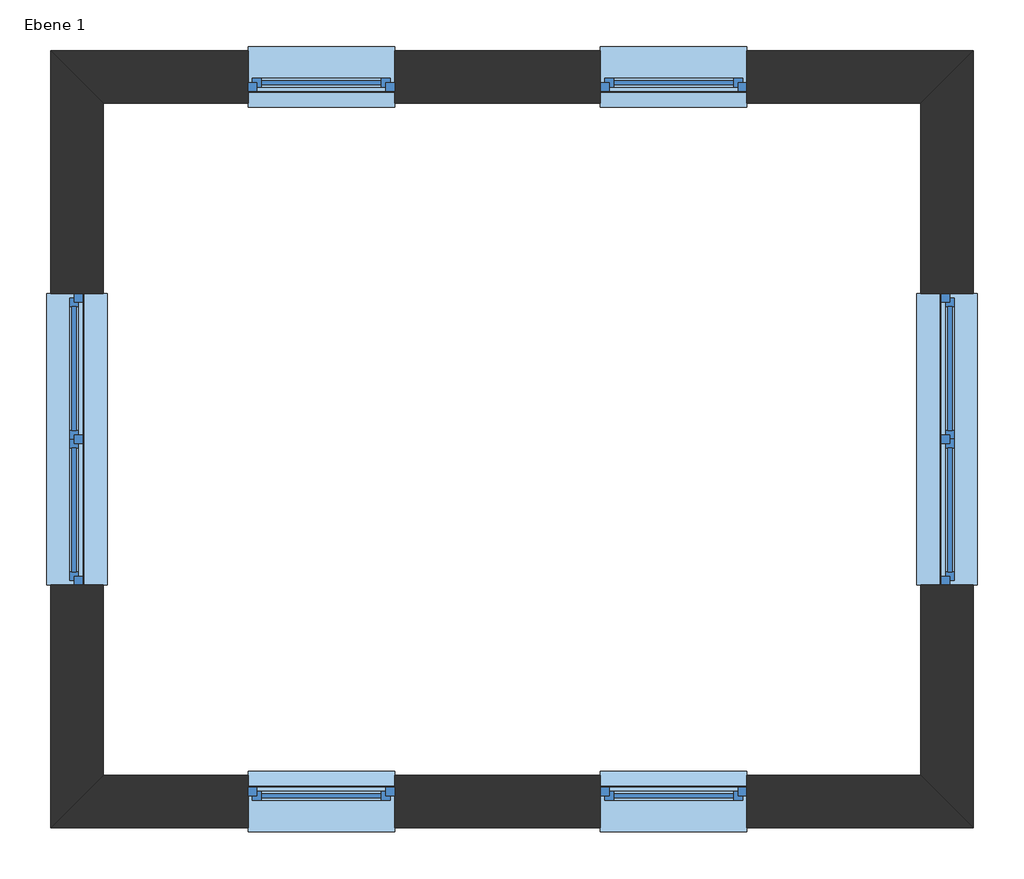
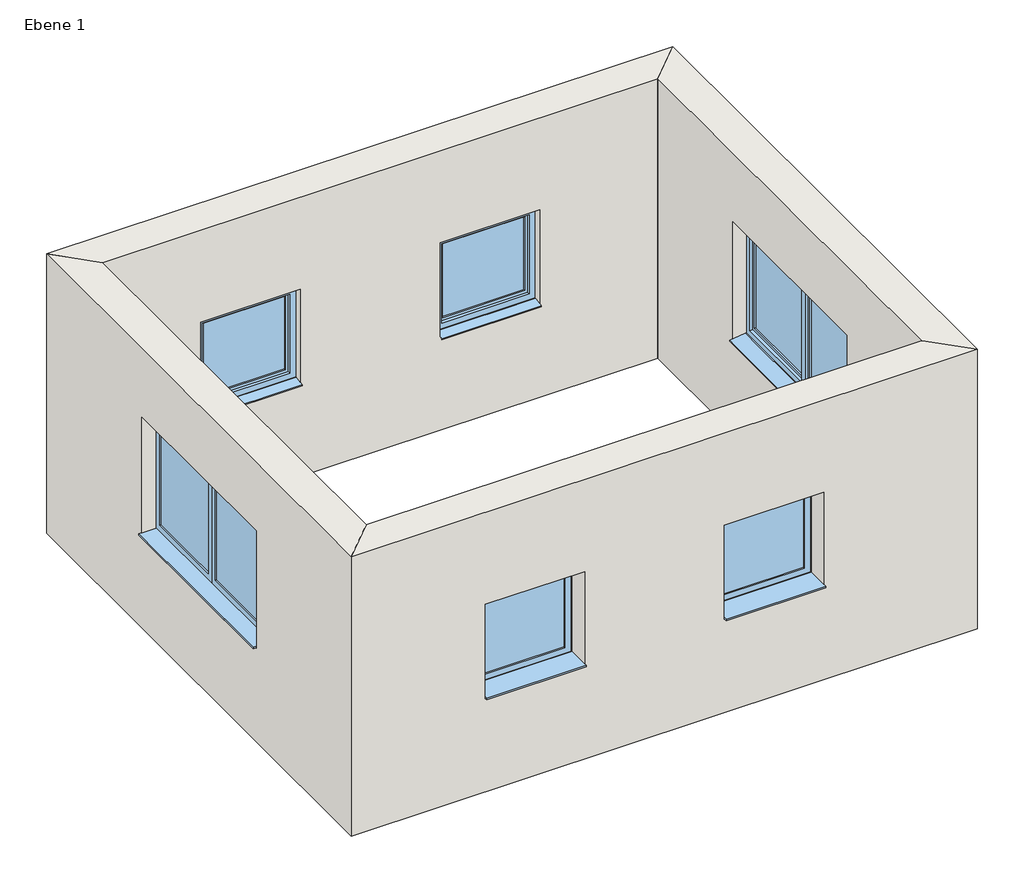
# One storey: 6 windows, 4 walls.
"""IFC4 building model written with IfcOpenShell, lengths in millimetres."""

import ifcopenshell
import ifcopenshell.guid

model = None  # the IFC model being written
_history = None  # IfcOwnerHistory: only IFC2X3 demands one
_inside = {}  # id of a spatial element -> (the spatial element, [elements in it])
_under = {}  # id of a project, library or spatial element -> (it, [spatial elements below it])
_declared = {}  # id of a project -> (the project, [libraries it declares])
_typed = {}  # id of a type object -> (the type object, [elements of that type])
_made_of = {}  # id of a material, layer set ... -> (it, [elements and type objects made of it])


def new_model(schema):
    """Start an empty IFC model of exactly this schema.

    Asked for "IFC4X3", IfcOpenShell would pick the latest addendum, in which some entities
    have other attributes; the version numbers below select the first issue.
    IFC2X3 requires an IfcOwnerHistory on every rooted entity: one is made here for all.
    """
    global model, _history
    if schema == "IFC4X3":
        model = ifcopenshell.file(schema_version=(4, 3, 0, 0))
    else:
        model = ifcopenshell.file(schema=schema)
    _inside.clear()
    _under.clear()
    _declared.clear()
    _typed.clear()
    _made_of.clear()
    _history = None
    if model.schema == "IFC2X3":
        org = make("IfcOrganization", Name="unknown")
        user = make(
            "IfcPersonAndOrganization",
            ThePerson=make("IfcPerson", FamilyName="unknown"),
            TheOrganization=org,
        )
        app = make(
            "IfcApplication",
            ApplicationDeveloper=org,
            Version="unknown",
            ApplicationFullName="unknown",
            ApplicationIdentifier="unknown",
        )
        _history = make(
            "IfcOwnerHistory",
            OwningUser=user,
            OwningApplication=app,
            ChangeAction="ADDED",
            CreationDate=0,
        )
    return model


def make(cls, **values):
    """One entity of the class cls with the attributes given. An attribute that is None is left unset."""
    return model.create_entity(
        cls, **{name: value for name, value in values.items() if value is not None}
    )


def rooted(cls, **values):
    """An entity with a GlobalId (a new one), such as an element, a storey or a relation."""
    return make(cls, GlobalId=ifcopenshell.guid.new(), OwnerHistory=_history, **values)


def si_unit(unit_type, name, prefix=None):
    """IfcSIUnit, for example si_unit("LENGTHUNIT", "METRE", prefix="MILLI")."""
    return make("IfcSIUnit", UnitType=unit_type, Prefix=prefix, Name=name)


def assignment(units):
    """IfcUnitAssignment: the units of a project."""
    return None if units is None else make("IfcUnitAssignment", Units=units)


def point(xyz):
    """IfcCartesianPoint."""
    return None if xyz is None else make("IfcCartesianPoint", Coordinates=xyz)


def direction(xyz):
    """IfcDirection."""
    return None if xyz is None else make("IfcDirection", DirectionRatios=xyz)


def frame(location, z_axis=None, x_axis=None):
    """IfcAxis2Placement3D, a coordinate frame: its origin and axes. An axis left out is left unset."""
    return make(
        "IfcAxis2Placement3D",
        Location=point(location),
        Axis=direction(z_axis),
        RefDirection=direction(x_axis),
    )


def origin():
    """The frame at (0, 0, 0) with its axes left unset."""
    return frame((0.0, 0.0, 0.0))


def place(relative_to, where):
    """IfcLocalPlacement: puts the frame where relative to a parent placement (None: the world)."""
    return make(
        "IfcLocalPlacement", PlacementRelTo=relative_to, RelativePlacement=where
    )


def context(
    kind, dimensions, precision=None, world=None, true_north=None, identifier=None
):
    """IfcGeometricRepresentationContext, for example the 3D "Model" context."""
    return make(
        "IfcGeometricRepresentationContext",
        ContextIdentifier=identifier,
        ContextType=kind,
        CoordinateSpaceDimension=dimensions,
        Precision=precision,
        WorldCoordinateSystem=world,
        TrueNorth=true_north,
    )


def project(units=None, contexts=None):
    """IfcProject with its units and contexts."""
    return rooted(
        "IfcProject",
        Name="project",
        RepresentationContexts=contexts,
        UnitsInContext=assignment(units),
    )


def spatial(cls, under=None, at=None, **own):
    """A site, building, storey or space (cls), placed at a placement, below another one or the project."""
    s = rooted(cls, ObjectPlacement=at, **own)
    if under is not None:
        _under.setdefault(under.id(), (under, []))[1].append(s)
    return s


def polyline(points):
    """IfcPolyline through the points."""
    return make("IfcPolyline", Points=[point(p) for p in points])


def outline(outer, holes=None, kind="AREA"):
    """IfcArbitraryClosedProfileDef: a profile drawn as a closed curve; with holes, ...WithVoids."""
    if holes is None:
        return make("IfcArbitraryClosedProfileDef", ProfileType=kind, OuterCurve=outer)
    return make(
        "IfcArbitraryProfileDefWithVoids",
        ProfileType=kind,
        OuterCurve=outer,
        InnerCurves=holes,
    )


def extrude(swept, where, along, depth):
    """IfcExtrudedAreaSolid: the profile swept, set in the frame where, extruded along a direction by depth."""
    return make(
        "IfcExtrudedAreaSolid",
        SweptArea=swept,
        Position=where,
        ExtrudedDirection=direction(along),
        Depth=depth,
    )


def faces_of(points, faces, orient=None, outer=None):
    """IfcFace entities. A face is a list of loops; a loop is a list of indices into points, from 0.

    orient and outer hold one flag for each loop. By default every Orientation is true, the
    first loop of a face is its IfcFaceOuterBound and the others are IfcFaceBound.
    """
    made = []
    for i, loops in enumerate(faces):
        bounds = []
        for j, loop in enumerate(loops):
            is_outer = j == 0 if outer is None else outer[i][j]
            bounds.append(
                make(
                    "IfcFaceOuterBound" if is_outer else "IfcFaceBound",
                    Bound=make("IfcPolyLoop", Polygon=[points[k] for k in loop]),
                    Orientation=True if orient is None else orient[i][j],
                )
            )
        made.append(make("IfcFace", Bounds=bounds))
    return made


def faceted_brep(points, faces, orient=None, outer=None, voids=None):
    """IfcFacetedBrep: a solid bounded by flat faces; with voids (closed shells), ...WithVoids."""
    shared = [point(p) for p in points]
    hull = make("IfcClosedShell", CfsFaces=faces_of(shared, faces, orient, outer))
    if voids is None:
        return make("IfcFacetedBrep", Outer=hull)
    return make(
        "IfcFacetedBrepWithVoids",
        Outer=hull,
        Voids=[
            make(cls, CfsFaces=faces_of(shared, fs, o, b)) for cls, fs, o, b in voids
        ],
    )


def shape(context_of_items, identifier, shape_type, items):
    """IfcShapeRepresentation: the items that make up one representation, for example the "Body"."""
    return make(
        "IfcShapeRepresentation",
        ContextOfItems=context_of_items,
        RepresentationIdentifier=identifier,
        RepresentationType=shape_type,
        Items=items,
    )


def source(mapping_origin, context_of_items, identifier, shape_type, items):
    """IfcRepresentationMap: a shape defined once, which mapped items show again and again."""
    return make(
        "IfcRepresentationMap",
        MappingOrigin=mapping_origin,
        MappedRepresentation=shape(context_of_items, identifier, shape_type, items),
    )


def transform(
    local_origin,
    x_axis=None,
    y_axis=None,
    z_axis=None,
    scale=None,
    scale2=None,
    scale3=None,
    uniform=True,
):
    """IfcCartesianTransformationOperator3D, or its non-uniform kind. x_axis, y_axis, z_axis: its Axis1, 2, 3."""
    if uniform:
        return make(
            "IfcCartesianTransformationOperator3D",
            Axis1=direction(x_axis),
            Axis2=direction(y_axis),
            LocalOrigin=point(local_origin),
            Scale=scale,
            Axis3=direction(z_axis),
        )
    return make(
        "IfcCartesianTransformationOperator3DnonUniform",
        Axis1=direction(x_axis),
        Axis2=direction(y_axis),
        LocalOrigin=point(local_origin),
        Scale=scale,
        Axis3=direction(z_axis),
        Scale2=scale2,
        Scale3=scale3,
    )


def mapped(mapping_source, mapping_target):
    """IfcMappedItem: shows the shape of a source again, moved by a transform."""
    return make(
        "IfcMappedItem", MappingSource=mapping_source, MappingTarget=mapping_target
    )


def made_of(thing, what):
    """Note that an element or type object is made of a material, layer set ...; save() writes the relation."""
    if what is not None:
        _made_of.setdefault(what.id(), (what, []))[1].append(thing)
    return thing


def element(
    cls,
    number,
    at=None,
    inside=None,
    cuts=None,
    type_object=None,
    material=None,
    context=None,
    identifier="Body",
    shape_type=None,
    held_by="IfcProductDefinitionShape",
    body=None,
    shapes=None,
    **own,
):
    """One element of the class cls, such as IfcWall. Its Tag is "e" and its number.

    at: its placement. inside: the storey or other place that contains it. cuts: it is an
    opening in that element (IfcRelVoidsElement). A single representation is given by context,
    identifier, shape_type and body (its items); several are given by shapes. held_by: the class
    of the entity that holds the representations. save() writes the other relations.
    """
    e = rooted(cls, Tag="e%d" % number, ObjectPlacement=at, **own)
    if body is not None:
        shapes = [shape(context, identifier, shape_type, body)]
    if shapes is not None:
        e.Representation = make(held_by, Representations=shapes)
    if inside is not None:
        _inside.setdefault(inside.id(), (inside, []))[1].append(e)
    if cuts is not None:
        rooted(
            "IfcRelVoidsElement", RelatingBuildingElement=cuts, RelatedOpeningElement=e
        )
    if type_object is not None:
        _typed.setdefault(type_object.id(), (type_object, []))[1].append(e)
    return made_of(e, material)


def aggregate(whole, parts):
    """IfcRelAggregates: a whole, such as a stair, and the parts it consists of."""
    return rooted("IfcRelAggregates", RelatingObject=whole, RelatedObjects=parts)


def save(model, path):
    """Write the relations noted so far, then the file.

    IfcRelAggregates (storeys below a building ...), IfcRelContainedInSpatialStructure (elements
    in a storey), IfcRelDefinesByType, IfcRelAssociatesMaterial and IfcRelDeclares: one each for
    every whole, place, type object, material and project.
    """
    for whole, parts in _under.values():
        aggregate(whole, parts)
    for where, things in _inside.values():
        rooted(
            "IfcRelContainedInSpatialStructure",
            RelatedElements=things,
            RelatingStructure=where,
        )
    for kind, things in _typed.values():
        rooted("IfcRelDefinesByType", RelatedObjects=things, RelatingType=kind)
    for what, things in _made_of.values():
        rooted("IfcRelAssociatesMaterial", RelatedObjects=things, RelatingMaterial=what)
    for by, libraries in _declared.values():
        rooted("IfcRelDeclares", RelatingContext=by, RelatedDefinitions=libraries)
    model.write(path)


def fenster_1_flg_variabel_fenster_1_flg_variabel_3_8a378bad(model_context):
    return source(origin(), model_context, "Body", "SolidModel", [
        extrude(outline(polyline([(2010.0, 505.0), (2010.0, -505.0), (1000.0, -505.0), (1000.0, 505.0), (2010.0, 505.0)]), holes=[polyline([(1930.0, 445.0), (1080.0, 445.0), (1080.0, -445.0), (1930.0, -445.0), (1930.0, 445.0)])]), frame((0.0, 40.0, 0.0), z_axis=(0.0, 1.0, 0.0), x_axis=(0.0, 0.0, 1.0)), (0.0, 0.0, 1.0), 60.0),
        faceted_brep([(475.0, 40.0, 1960.0), (475.0, 10.0, 1960.0), (475.0, 10.0, 1050.0), (475.0, 40.0, 1050.0), (-475.0, 10.0, 1960.0), (-475.0, 10.0, 1050.0), (415.0, 10.0, 1110.0), (-415.0, 10.0, 1110.0), (-415.0, 10.0, 1900.0), (415.0, 10.0, 1900.0), (-475.0, 40.0, 1050.0), (-475.0, 40.0, 1960.0), (445.0, 40.0, 1930.0), (-445.0, 40.0, 1930.0), (-445.0, 40.0, 1080.0), (445.0, 40.0, 1080.0), (445.0, 70.0, 1930.0), (445.0, 70.0, 1080.0), (-445.0, 70.0, 1080.0), (-445.0, 70.0, 1930.0), (415.0, 70.0, 1900.0), (-415.0, 70.0, 1900.0), (-415.0, 70.0, 1110.0), (415.0, 70.0, 1110.0)], [[[0, 1, 2, 3]], [[1, 4, 5, 2], [6, 7, 8, 9]], [[3, 2, 5, 10]], [[3, 10, 11, 0], [12, 13, 14, 15]], [[16, 12, 15, 17]], [[17, 15, 14, 18]], [[17, 18, 19, 16], [20, 21, 22, 23]], [[9, 20, 23, 6]], [[6, 23, 22, 7]], [[10, 5, 4, 11]], [[18, 14, 13, 19]], [[7, 22, 21, 8]], [[11, 4, 1, 0]], [[19, 13, 12, 16]], [[8, 21, 20, 9]]]),
        extrude(outline(polyline([(-505.0, -210.0), (-505.0, 40.0), (505.0, 40.0), (505.0, -210.0), (-505.0, -210.0)])), frame((0.0, 0.0, 1005.0), z_axis=(0.0, 0.0, 1.0), x_axis=(1.0, 0.0, 0.0)), (0.0, 0.0, 1.0), 15.0),
        extrude(outline(polyline([(110.0221543, 1020.0), (210.0, 1000.0), (210.0, 990.0), (208.0, 990.0), (208.0, 998.3604634), (109.8240723, 1018.0), (100.0, 1018.0), (100.0, 1020.0), (110.0221543, 1020.0)])), frame((-505.0, 0.0, 0.0), z_axis=(1.0, 0.0, 0.0), x_axis=(0.0, 1.0, 0.0)), (0.0, 0.0, 1.0), 1010.0),
        extrude(outline(polyline([(415.0, 25.0), (-415.0, 25.0), (-415.0, 55.0), (415.0, 55.0), (415.0, 25.0)])), frame((0.0, 0.0, 1110.0), z_axis=(0.0, 0.0, 1.0), x_axis=(1.0, 0.0, 0.0)), (0.0, 0.0, 1.0), 790.0),
    ])


def fenster_2_flg_variabel_fenster_2_flg_variabel_3_03287464(model_context):
    return source(origin(), model_context, "Body", "SolidModel", [
        extrude(outline(polyline([(60.0, -5.0), (915.0, -5.0), (915.0, -35.0), (60.0, -35.0), (60.0, -5.0)])), frame((0.0, 0.0, 1110.0), z_axis=(0.0, 0.0, 1.0), x_axis=(1.0, 0.0, 0.0)), (0.0, 0.0, 1.0), 1040.0),
        extrude(outline(polyline([(-915.0, -5.0), (-60.0, -5.0), (-60.0, -35.0), (-915.0, -35.0), (-915.0, -5.0)])), frame((0.0, 0.0, 1110.0), z_axis=(0.0, 0.0, 1.0), x_axis=(1.0, 0.0, 0.0)), (0.0, 0.0, 1.0), 1040.0),
        extrude(outline(polyline([(-1005.0, -210.0), (-1005.0, -20.0), (1005.0, -20.0), (1005.0, -210.0), (-1005.0, -210.0)])), frame((0.0, 0.0, 1005.0), z_axis=(0.0, 0.0, 1.0), x_axis=(1.0, 0.0, 0.0)), (0.0, 0.0, 1.0), 15.0),
        extrude(outline(polyline([(50.0221543, 1020.0), (210.0, 1000.0), (210.0, 990.0), (208.0, 990.0), (208.0, 998.3604634), (49.8240723, 1018.0), (40.0, 1018.0), (40.0, 1020.0), (50.0221543, 1020.0)])), frame((-1005.0, 0.0, 0.0), z_axis=(1.0, 0.0, 0.0), x_axis=(0.0, 1.0, 0.0)), (0.0, 0.0, 1.0), 2010.0),
        extrude(outline(polyline([(30.0, -20.0), (-30.0, -20.0), (-30.0, 40.0), (30.0, 40.0), (30.0, -20.0)])), frame((0.0, 0.0, 1080.0), z_axis=(0.0, 0.0, 1.0), x_axis=(1.0, 0.0, 0.0)), (0.0, 0.0, 1.0), 1100.0),
        extrude(outline(polyline([(2260.0, -1005.0), (1000.0, -1005.0), (1000.0, 1005.0), (2260.0, 1005.0), (2260.0, -1005.0)]), holes=[polyline([(2180.0, -945.0), (2180.0, 945.0), (1080.0, 945.0), (1080.0, -945.0), (2180.0, -945.0)])]), frame((0.0, -20.0, 0.0), z_axis=(0.0, 1.0, 0.0), x_axis=(0.0, 0.0, 1.0)), (0.0, 0.0, 1.0), 60.0),
        faceted_brep([(-945.0, -20.0, 1080.0), (-945.0, 10.0, 1080.0), (-30.0, 10.0, 1080.0), (-30.0, -20.0, 1080.0), (-30.0, 10.0, 2180.0), (-30.0, -20.0, 2180.0), (-945.0, 10.0, 2180.0), (-60.0, 10.0, 2150.0), (-915.0, 10.0, 2150.0), (-915.0, 10.0, 1110.0), (-60.0, 10.0, 1110.0), (0.0, -20.0, 1050.0), (-975.0, -20.0, 1050.0), (-975.0, -20.0, 2210.0), (0.0, -20.0, 2210.0), (-945.0, -20.0, 2180.0), (-975.0, -50.0, 1050.0), (0.0, -50.0, 1050.0), (0.0, -50.0, 2210.0), (-975.0, -50.0, 2210.0), (-60.0, -50.0, 1110.0), (-915.0, -50.0, 1110.0), (-915.0, -50.0, 2150.0), (-60.0, -50.0, 2150.0)], [[[0, 1, 2, 3]], [[3, 2, 4, 5]], [[2, 1, 6, 4], [7, 8, 9, 10]], [[11, 12, 13, 14], [5, 15, 0, 3]], [[16, 12, 11, 17]], [[17, 11, 14, 18]], [[18, 19, 16, 17], [20, 21, 22, 23]], [[9, 21, 20, 10]], [[10, 20, 23, 7]], [[15, 6, 1, 0]], [[19, 13, 12, 16]], [[8, 22, 21, 9]], [[5, 4, 6, 15]], [[18, 14, 13, 19]], [[7, 23, 22, 8]]]),
        faceted_brep([(30.0, -20.0, 1080.0), (30.0, 10.0, 1080.0), (945.0, 10.0, 1080.0), (945.0, -20.0, 1080.0), (945.0, 10.0, 2180.0), (945.0, -20.0, 2180.0), (30.0, 10.0, 2180.0), (915.0, 10.0, 2150.0), (60.0, 10.0, 2150.0), (60.0, 10.0, 1110.0), (915.0, 10.0, 1110.0), (975.0, -20.0, 1050.0), (0.0, -20.0, 1050.0), (0.0, -20.0, 2210.0), (975.0, -20.0, 2210.0), (30.0, -20.0, 2180.0), (0.0, -50.0, 1050.0), (975.0, -50.0, 1050.0), (975.0, -50.0, 2210.0), (0.0, -50.0, 2210.0), (915.0, -50.0, 1110.0), (60.0, -50.0, 1110.0), (60.0, -50.0, 2150.0), (915.0, -50.0, 2150.0)], [[[0, 1, 2, 3]], [[3, 2, 4, 5]], [[2, 1, 6, 4], [7, 8, 9, 10]], [[11, 12, 13, 14], [5, 15, 0, 3]], [[16, 12, 11, 17]], [[17, 11, 14, 18]], [[18, 19, 16, 17], [20, 21, 22, 23]], [[9, 21, 20, 10]], [[10, 20, 23, 7]], [[15, 6, 1, 0]], [[19, 13, 12, 16]], [[8, 22, 21, 9]], [[5, 4, 6, 15]], [[18, 14, 13, 19]], [[7, 23, 22, 8]]]),
    ])


model = new_model("IFC4")

# Units and contexts
model_context = context("Model", 3, world=origin())
ifc_project = project(units=[si_unit("LENGTHUNIT", "METRE", prefix="MILLI")], contexts=[model_context])

# Site, building, storey
site = spatial("IfcSite", under=ifc_project)
building = spatial("IfcBuilding", under=site)
storey = spatial("IfcBuildingStorey", under=building, Name="Ebene 1", Elevation=3000.0)

# Walls
placement = place(None, origin())
element("IfcWall", 1, ObjectType="MW 24.0 WD 12.0", at=placement, inside=storey, context=model_context, shape_type="Brep", body=[
    faceted_brep([(-6003.5987005, 5004.2257101, 3000.0), (-363.5987005, 5004.2257101, 3000.0), (-363.5987005, 5004.2257101, 6000.0), (-6003.5987005, 5004.2257101, 6000.0), (-1563.5987005, 5004.2257101, 4000.0), (-2573.5987005, 5004.2257101, 4000.0), (-2573.5987005, 5004.2257101, 5010.0), (-1563.5987005, 5004.2257101, 5010.0), (-3993.5987005, 5004.2257101, 4000.0), (-5003.5987005, 5004.2257101, 4000.0), (-5003.5987005, 5004.2257101, 5010.0), (-3993.5987005, 5004.2257101, 5010.0), (-6363.5987005, 5364.2257101, 3000.0), (-6363.5987005, 5364.2257101, 6000.0), (-3.5987005, 5364.2257101, 6000.0), (-3.5987005, 5364.2257101, 3000.0), (-1563.5987005, 5364.2257101, 4000.0), (-1563.5987005, 5364.2257101, 5010.0), (-2573.5987005, 5364.2257101, 5010.0), (-2573.5987005, 5364.2257101, 4000.0), (-3993.5987005, 5364.2257101, 4000.0), (-3993.5987005, 5364.2257101, 5010.0), (-5003.5987005, 5364.2257101, 5010.0), (-5003.5987005, 5364.2257101, 4000.0)], [[[0, 1, 2, 3], [4, 5, 6, 7], [8, 9, 10, 11]], [[12, 13, 14, 15], [16, 17, 18, 19], [20, 21, 22, 23]], [[1, 0, 12, 15]], [[3, 2, 14, 13]], [[2, 1, 15, 14]], [[0, 3, 13, 12]], [[17, 16, 4, 7]], [[18, 17, 7, 6]], [[19, 18, 6, 5]], [[16, 19, 5, 4]], [[21, 20, 8, 11]], [[22, 21, 11, 10]], [[23, 22, 10, 9]], [[20, 23, 9, 8]]]),
])
element("IfcWall", 2, ObjectType="MW 24.0 WD 12.0", at=placement, inside=storey, context=model_context, shape_type="Brep", body=[
    faceted_brep([(-363.5987005, 5004.2257101, 3000.0), (-363.5987005, 364.2257101, 3000.0), (-363.5987005, 364.2257101, 6000.0), (-363.5987005, 5004.2257101, 6000.0), (-363.5987005, 1679.2257101, 4000.0), (-363.5987005, 3689.2257101, 4000.0), (-363.5987005, 3689.2257101, 5260.0), (-363.5987005, 1679.2257101, 5260.0), (-3.5987005, 5364.2257101, 3000.0), (-3.5987005, 5364.2257101, 6000.0), (-3.5987005, 4.2257101, 6000.0), (-3.5987005, 4.2257101, 3000.0), (-3.5987005, 1679.2257101, 4000.0), (-3.5987005, 1679.2257101, 5260.0), (-3.5987005, 3689.2257101, 5260.0), (-3.5987005, 3689.2257101, 4000.0)], [[[0, 1, 2, 3], [4, 5, 6, 7]], [[8, 9, 10, 11], [12, 13, 14, 15]], [[1, 0, 8, 11]], [[3, 2, 10, 9]], [[0, 3, 9, 8]], [[2, 1, 11, 10]], [[13, 12, 4, 7]], [[14, 13, 7, 6]], [[15, 14, 6, 5]], [[12, 15, 5, 4]]]),
])
element("IfcWall", 3, ObjectType="MW 24.0 WD 12.0", at=placement, inside=storey, context=model_context, shape_type="Brep", body=[
    faceted_brep([(-363.5987005, 364.2257101, 3000.0), (-6003.5987005, 364.2257101, 3000.0), (-6003.5987005, 364.2257101, 6000.0), (-363.5987005, 364.2257101, 6000.0), (-2573.5987005, 364.2257101, 4000.0), (-1563.5987005, 364.2257101, 4000.0), (-1563.5987005, 364.2257101, 5010.0), (-2573.5987005, 364.2257101, 5010.0), (-5003.5987005, 364.2257101, 4000.0), (-3993.5987005, 364.2257101, 4000.0), (-3993.5987005, 364.2257101, 5010.0), (-5003.5987005, 364.2257101, 5010.0), (-3.5987005, 4.2257101, 3000.0), (-3.5987005, 4.2257101, 6000.0), (-6363.5987005, 4.2257101, 6000.0), (-6363.5987005, 4.2257101, 3000.0), (-2573.5987005, 4.2257101, 4000.0), (-2573.5987005, 4.2257101, 5010.0), (-1563.5987005, 4.2257101, 5010.0), (-1563.5987005, 4.2257101, 4000.0), (-5003.5987005, 4.2257101, 4000.0), (-5003.5987005, 4.2257101, 5010.0), (-3993.5987005, 4.2257101, 5010.0), (-3993.5987005, 4.2257101, 4000.0)], [[[0, 1, 2, 3], [4, 5, 6, 7], [8, 9, 10, 11]], [[12, 13, 14, 15], [16, 17, 18, 19], [20, 21, 22, 23]], [[1, 0, 12, 15]], [[3, 2, 14, 13]], [[0, 3, 13, 12]], [[2, 1, 15, 14]], [[17, 16, 4, 7]], [[18, 17, 7, 6]], [[19, 18, 6, 5]], [[16, 19, 5, 4]], [[21, 20, 8, 11]], [[22, 21, 11, 10]], [[23, 22, 10, 9]], [[20, 23, 9, 8]]]),
])
element("IfcWall", 4, ObjectType="MW 24.0 WD 12.0", at=placement, inside=storey, context=model_context, shape_type="Brep", body=[
    faceted_brep([(-6003.5987005, 364.2257101, 3000.0), (-6003.5987005, 5004.2257101, 3000.0), (-6003.5987005, 5004.2257101, 6000.0), (-6003.5987005, 364.2257101, 6000.0), (-6003.5987005, 3689.2257101, 4000.0), (-6003.5987005, 1679.2257101, 4000.0), (-6003.5987005, 1679.2257101, 5260.0), (-6003.5987005, 3689.2257101, 5260.0), (-6363.5987005, 4.2257101, 3000.0), (-6363.5987005, 4.2257101, 6000.0), (-6363.5987005, 5364.2257101, 6000.0), (-6363.5987005, 5364.2257101, 3000.0), (-6363.5987005, 3689.2257101, 4000.0), (-6363.5987005, 3689.2257101, 5260.0), (-6363.5987005, 1679.2257101, 5260.0), (-6363.5987005, 1679.2257101, 4000.0)], [[[0, 1, 2, 3], [4, 5, 6, 7]], [[8, 9, 10, 11], [12, 13, 14, 15]], [[1, 0, 8, 11]], [[3, 2, 10, 9]], [[2, 1, 11, 10]], [[0, 3, 9, 8]], [[13, 12, 4, 7]], [[14, 13, 7, 6]], [[15, 14, 6, 5]], [[12, 15, 5, 4]]]),
])

# Windows
fenster_1_flg_variabel_fenster_1_flg_variabel_3_shape = fenster_1_flg_variabel_fenster_1_flg_variabel_3_8a378bad(model_context)
element("IfcWindow", 5, ObjectType="Fenster 1-flg - Variabel : Fenster 1-flg - Variabel 3", at=placement, inside=storey, context=model_context, shape_type="MappedRepresentation", body=[
    mapped(fenster_1_flg_variabel_fenster_1_flg_variabel_3_shape, transform((-2068.5987005, 184.2257101, 3000.0), x_axis=(1.0, 0.0, 0.0), y_axis=(0.0, 1.0, 0.0), z_axis=(0.0, 0.0, 1.0))),
])
element("IfcWindow", 6, ObjectType="Fenster 1-flg - Variabel : Fenster 1-flg - Variabel 3", at=placement, inside=storey, context=model_context, shape_type="MappedRepresentation", body=[
    mapped(fenster_1_flg_variabel_fenster_1_flg_variabel_3_shape, transform((-4498.5987005, 184.2257101, 3000.0), x_axis=(1.0, 0.0, 0.0), y_axis=(0.0, 1.0, 0.0), z_axis=(0.0, 0.0, 1.0))),
])
element("IfcWindow", 7, ObjectType="Fenster 1-flg - Variabel : Fenster 1-flg - Variabel 3", at=placement, inside=storey, context=model_context, shape_type="MappedRepresentation", body=[
    mapped(fenster_1_flg_variabel_fenster_1_flg_variabel_3_shape, transform((-2068.5987005, 5184.2257101, 3000.0), x_axis=(-1.0, 0.0, 0.0), y_axis=(0.0, -1.0, 0.0), z_axis=(0.0, 0.0, 1.0))),
])
element("IfcWindow", 8, ObjectType="Fenster 1-flg - Variabel : Fenster 1-flg - Variabel 3", at=placement, inside=storey, context=model_context, shape_type="MappedRepresentation", body=[
    mapped(fenster_1_flg_variabel_fenster_1_flg_variabel_3_shape, transform((-4498.5987005, 5184.2257101, 3000.0), x_axis=(-1.0, 0.0, 0.0), y_axis=(0.0, -1.0, 0.0), z_axis=(0.0, 0.0, 1.0))),
])
fenster_2_flg_variabel_fenster_2_flg_variabel_3_shape = fenster_2_flg_variabel_fenster_2_flg_variabel_3_03287464(model_context)
element("IfcWindow", 9, ObjectType="Fenster 2-flg - Variabel : Fenster 2-flg - Variabel 3", at=placement, inside=storey, context=model_context, shape_type="MappedRepresentation", body=[
    mapped(fenster_2_flg_variabel_fenster_2_flg_variabel_3_shape, transform((-183.5987005, 2684.2257101, 3000.0), x_axis=(0.0, 1.0, 0.0), y_axis=(-1.0, 0.0, 0.0), z_axis=(0.0, 0.0, 1.0))),
])
element("IfcWindow", 10, ObjectType="Fenster 2-flg - Variabel : Fenster 2-flg - Variabel 3", at=placement, inside=storey, context=model_context, shape_type="MappedRepresentation", body=[
    mapped(fenster_2_flg_variabel_fenster_2_flg_variabel_3_shape, transform((-6183.5987005, 2684.2257101, 3000.0), x_axis=(0.0, -1.0, 0.0), y_axis=(1.0, 0.0, 0.0), z_axis=(0.0, 0.0, 1.0))),
])

save(model, "model.ifc")

# Revit data of these elements
# Type "MW 24.0 WD 12.0"
#   Type Comments = "Mehrschaliges Mauerwerk"
#   Description = "Mauerwerk 24.0 cm, Wärmedämmung 12.0 cm"
#   Layers, outside or top first: 0.120 m "Wärmedämmung - hart" (function 3); 0.240 m "Mauerwerk - Ziegel, verputzt" (function 1)
# Type "Fenster 1-flg - Variabel : Fenster 1-flg - Variabel 3"
#   Type Mark = "52"
#   Operation = "SinglePanel"
#   Construction Type Id = "GSP4R"
#   Keynote = "16.05.01"
#   Analytic Construction = "1/8 Zoll Pilkington-Verglasung einfach"
#   Cost = 78.2
#   Visual Light Transmittance = 0.9
#   Höhe oberer  Rahmen = 0.080 m
#   Solar Heat Gain Coefficient = 0.86
#   Tiefe Flügel = 0.060 m
#   Rough Width [instance default] = 1.010 m
#   Rough Height [instance default] = 1.010 m
#   Rahmenhöhe unten = 0.080 m
#   Heat Transfer Coefficient (U) = 6.7069 W/(m²·K)
#   Rahmentiefe = 0.060 m
#   Rahmenbreite = 0.060 m
#   Height [instance default] = 1.010 m
#   Flügelbreite = 0.060 m
#   Einbautiefe (von außen) [instance default] = 0.080 m
#   Width [instance default] = 1.010 m
#   Define Thermal Properties by = 1
#   Öffnungsrichtung oben [instance default] = yes
#   Öffnungsrichtung in Draufsicht anzeigen [instance default] = no
#   Klappflügel [instance default] = no
#   Drehflügel 1 [instance default] = yes
#   Fensterflügel [instance default] = none
#   Innere Fensterbank [instance default] = none
#   Glas [instance default] = none
#   Bild [instance default] = none
#   Äußere Fensterbank [instance default] = none
#   Wall Closure = (empty or 0)
# Type "Fenster 2-flg - Variabel : Fenster 2-flg - Variabel 3"
#   Type Mark = "53"
#   Operation = "DoublePanelVertical"
#   Construction Type Id = "GSP4R"
#   Keynote = "16.05.01"
#   Analytic Construction = "1/8 Zoll Pilkington-Verglasung einfach"
#   Cost = 130.98
#   Visual Light Transmittance = 0.9
#   Solar Heat Gain Coefficient = 0.78
#   Rough Width [instance default] = 2.010 m
#   Rough Height [instance default] = 1.260 m
#   Heat Transfer Coefficient (U) = 3.6886 W/(m²·K)
#   Rahmentiefe = 0.060 m
#   Rahmenhöhe unten = 0.080 m
#   Höhe oberer  Rahmen = 0.080 m
#   Rahmenbreite = 0.060 m
#   Height [instance default] = 1.260 m
#   Tiefe Flügel = 0.060 m
#   Flügelbreite = 0.060 m
#   Einbautiefe (von außen) [instance default] = 0.140 m
#   Width [instance default] = 2.010 m
#   Define Thermal Properties by = 1
#   Öffnungsrichtung oben [instance default] = yes
#   Öffnungsrichtung in Draufsicht anzeigen [instance default] = no
#   Drehflügel 1 [instance default] = yes
#   Bild [instance default] = none
#   Glas [instance default] = none
#   Fensterflügel [instance default] = none
#   Äußere Fensterbank [instance default] = none
#   Innere Fensterbank [instance default] = none
#   Wall Closure = (empty or 0)
# Elements 1, 2, 3, 4 (IfcWall, "MW 24.0 WD 12.0")
#   Comments = ""
#   Top Offset = 0.000 m
#   Base Offset = 0.000 m
#   Unconnected Height = 3.000 m
#   wall height = 3.000 m
#   Phase Created = Phase 1
#   Base Constraint = Ebene 1
#   Materials on its faces: "Vorgabe - Wand", "Mauerwerk - Ziegel, verputzt", "Wärmedämmung - hart"
# Element 5 (IfcWindow, "Fenster 1-flg - Variabel : Fenster 1-flg - Variabel 3")
#   Mark = "2"
#   Rough Height = 1.010 m
#   Rough Width = 1.010 m
#   Height = 1.010 m
#   Einbautiefe (von außen) = 0.080 m
#   Width = 1.010 m
#   Öffnungsrichtung oben = yes
#   Öffnungsrichtung in Draufsicht anzeigen = no
#   Klappflügel = no
#   Drehflügel 1 = yes
#   Äußere Fensterbank = none
#   Innere Fensterbank = none
#   Glas = none
#   Fensterflügel = none
#   Bild = none
#   Phase Created = Phase 1
#   Materials on its faces: "Kunststoff - Weiß", "Holz - Birke", "Glas"
# Element 6 (IfcWindow, "Fenster 1-flg - Variabel : Fenster 1-flg - Variabel 3")
#   Mark = "3"
#   Rough Height = 1.010 m
#   Rough Width = 1.010 m
#   Height = 1.010 m
#   Einbautiefe (von außen) = 0.080 m
#   Width = 1.010 m
#   Öffnungsrichtung oben = yes
#   Öffnungsrichtung in Draufsicht anzeigen = no
#   Klappflügel = no
#   Drehflügel 1 = yes
#   Äußere Fensterbank = none
#   Innere Fensterbank = none
#   Glas = none
#   Fensterflügel = none
#   Bild = none
#   Phase Created = Phase 1
#   Materials on its faces: "Kunststoff - Weiß", "Holz - Birke", "Glas"
# Element 7 (IfcWindow, "Fenster 1-flg - Variabel : Fenster 1-flg - Variabel 3")
#   Mark = "4"
#   Rough Height = 1.010 m
#   Rough Width = 1.010 m
#   Height = 1.010 m
#   Einbautiefe (von außen) = 0.080 m
#   Width = 1.010 m
#   Öffnungsrichtung oben = yes
#   Öffnungsrichtung in Draufsicht anzeigen = no
#   Klappflügel = no
#   Drehflügel 1 = yes
#   Äußere Fensterbank = none
#   Innere Fensterbank = none
#   Glas = none
#   Fensterflügel = none
#   Bild = none
#   Phase Created = Phase 1
#   Materials on its faces: "Kunststoff - Weiß", "Holz - Birke", "Glas"
# Element 8 (IfcWindow, "Fenster 1-flg - Variabel : Fenster 1-flg - Variabel 3")
#   Mark = "5"
#   Rough Height = 1.010 m
#   Rough Width = 1.010 m
#   Height = 1.010 m
#   Einbautiefe (von außen) = 0.080 m
#   Width = 1.010 m
#   Öffnungsrichtung oben = yes
#   Öffnungsrichtung in Draufsicht anzeigen = no
#   Klappflügel = no
#   Drehflügel 1 = yes
#   Äußere Fensterbank = none
#   Innere Fensterbank = none
#   Glas = none
#   Fensterflügel = none
#   Bild = none
#   Phase Created = Phase 1
#   Materials on its faces: "Kunststoff - Weiß", "Holz - Birke", "Glas"
# Element 9 (IfcWindow, "Fenster 2-flg - Variabel : Fenster 2-flg - Variabel 3")
#   Mark = "8"
#   Rough Height = 1.260 m
#   Rough Width = 2.010 m
#   Height = 1.260 m
#   Einbautiefe (von außen) = 0.140 m
#   Width = 2.010 m
#   Öffnungsrichtung oben = yes
#   Öffnungsrichtung in Draufsicht anzeigen = no
#   Drehflügel 1 = yes
#   Äußere Fensterbank = none
#   Innere Fensterbank = none
#   Glas = none
#   Fensterflügel = none
#   Bild = none
#   Phase Created = Phase 1
#   Materials on its faces: "Kunststoff - Weiß", "Glas", "Holz - Birke"
# Element 10 (IfcWindow, "Fenster 2-flg - Variabel : Fenster 2-flg - Variabel 3")
#   Mark = "9"
#   Rough Height = 1.260 m
#   Rough Width = 2.010 m
#   Height = 1.260 m
#   Einbautiefe (von außen) = 0.140 m
#   Width = 2.010 m
#   Öffnungsrichtung oben = yes
#   Öffnungsrichtung in Draufsicht anzeigen = no
#   Drehflügel 1 = yes
#   Äußere Fensterbank = none
#   Innere Fensterbank = none
#   Glas = none
#   Fensterflügel = none
#   Bild = none
#   Phase Created = Phase 1
#   Materials on its faces: "Kunststoff - Weiß", "Glas", "Holz - Birke"
# Materials
#   "Wärmedämmung - hart": class "Stuck", colour RGB 255 255 255, transparency 0, Description = "Äußere Oberfläche", Cost = 0
#   "Mauerwerk - Ziegel, verputzt": class "Stuck", colour RGB 247 247 247, transparency 0, Cost = 0
#   "Vorgabe - Wand": class "Stuck", colour RGB 128 128 128, transparency 0, Description = "Äußere Oberfläche", Cost = 0
#   "Kunststoff - Weiß": class "Kunststoff", colour RGB 249 249 249, transparency 0, Cost = 0
#   "Holz - Birke": class "Holz", colour RGB 213 164 103, transparency 0, Cost = 0
#   "Glas": class "Glas", colour RGB 0 0 255, transparency 0.75, Comments = "Render-Darstellung nicht aktualisiert ", Cost = 0
